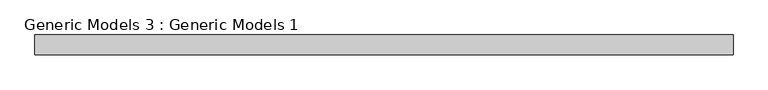
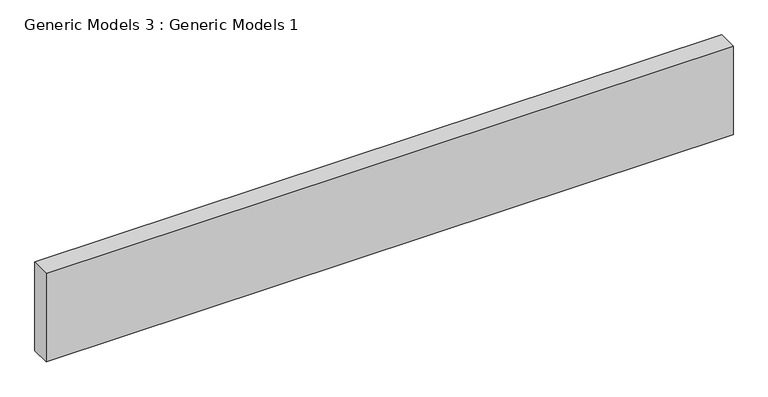
"""IFC4 building model written with IfcOpenShell, lengths in millimetres: proxy geometry, Generic Models 3 : Generic Models 1."""

from ifc_helpers import new_model, si_unit, frame, origin, place, context, project, spatial, polyline, outline, extrude, source, transform, mapped, element, save


def generic_models_3_generic_models_1_bac14a14(model_context):
    return source(origin(), model_context, "Body", "SweptSolid", [
        extrude(outline(polyline([(7162.6263704, 4561.4650592), (7162.6263704, 4599.5650592), (8508.8263704, 4599.5650592), (8508.8263704, 4561.4650592), (7162.6263704, 4561.4650592)])), frame((0.0, 0.0, 126586.996), z_axis=(0.0, 0.0, 1.0), x_axis=(1.0, 0.0, 0.0)), (0.0, 0.0, 1.0), 184.15),
    ])


if __name__ == "__main__":
    model = new_model("IFC4")
    model_context = context("Model", 3, world=origin())
    ifc_project = project(units=[si_unit("LENGTHUNIT", "METRE", prefix="MILLI")], contexts=[model_context])
    site = spatial("IfcSite", under=ifc_project)
    building = spatial("IfcBuilding", under=site)
    placement = place(None, origin())
    generic_models_3_generic_models_1_shape = generic_models_3_generic_models_1_bac14a14(model_context)
    element("IfcBuildingElementProxy", 1, Name="Generic Models 3 : Generic Models 1", ObjectType="Generic Models 3 : Generic Models 1", at=placement, inside=building, context=model_context, shape_type="MappedRepresentation", body=[
        mapped(generic_models_3_generic_models_1_shape, transform((0.0, 0.0, 0.0), x_axis=(1.0, 0.0, 0.0), y_axis=(0.0, 1.0, 0.0), z_axis=(0.0, 0.0, 1.0))),
    ])
    save(model, "model.ifc")

# Revit data of these elements
# Element 1 (IfcBuildingElementProxy, "Generic Models 3 : Generic Models 1")
#   Materials on its faces: "_STRUCTURAL MEMBER (SEE STRUCT. DWGS)"
# Materials
#   "_STRUCTURAL MEMBER (SEE STRUCT. DWGS)": class "Generic", colour RGB 209 182 141, transparency 0, Cost = 0
